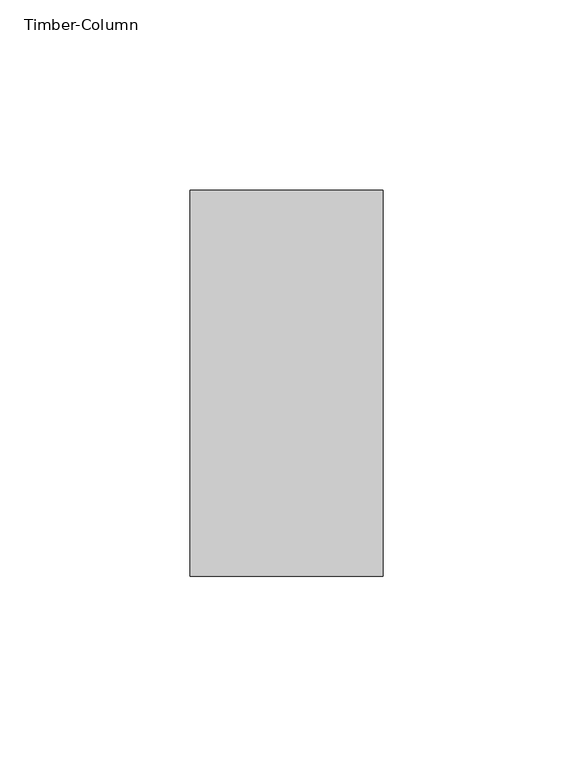
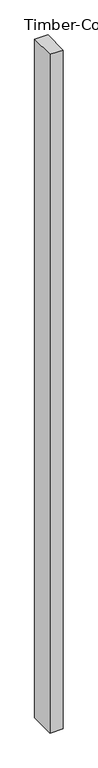
"""IFC4 building model written with IfcOpenShell, lengths in millimetres: column geometry, Timber-Column."""

from ifc_helpers import new_model, si_unit, origin, origin_with_axes, place, context, project, spatial, polyline, outline, extrude, source, transform, mapped, element, save


def timber_column_7e99ce9a(model_context):
    return source(origin(), model_context, "Body", "SweptSolid", [
        extrude(outline(polyline([(25.4, 50.8), (25.4, -50.8), (-25.4, -50.8), (-25.4, 50.8), (25.4, 50.8)])), origin_with_axes(), (0.0, 0.0, 1.0), 2768.6),
    ])


if __name__ == "__main__":
    model = new_model("IFC4")
    model_context = context("Model", 3, world=origin())
    ifc_project = project(units=[si_unit("LENGTHUNIT", "METRE", prefix="MILLI")], contexts=[model_context])
    site = spatial("IfcSite", under=ifc_project)
    building = spatial("IfcBuilding", under=site)
    placement = place(None, origin())
    timber_column_shape = timber_column_7e99ce9a(model_context)
    element("IfcColumn", 1, ObjectType="Timber-Column : BLDG 6241 Wall Struds 2\"x4\"", at=placement, inside=building, context=model_context, shape_type="MappedRepresentation", body=[
        mapped(timber_column_shape, transform((0.0, 0.0, 0.0), x_axis=(1.0, 0.0, 0.0), y_axis=(0.0, 1.0, 0.0), z_axis=(0.0, 0.0, 1.0))),
    ])
    save(model, "model.ifc")

# Revit data of these elements
# Type "Timber-Column : BLDG 6241 Wall Struds 2\"x4\""
#   Assembly Code = "B10"
#   A = 0.140625 SF
#   b = 0' - 2"
#   d = 0' - 4"
#   Structural Material [instance default] = Softwood, Lumber
# Element 1 (IfcColumn, "Timber-Column : BLDG 6241 Wall Struds 2\"x4\"")
#   Materials on its faces: "Softwood, Lumber"
# Materials
#   "Softwood, Lumber": class "Wood", colour RGB 223 192 134, transparency 0, Description = "Pinus Echinata", Cost = 0
